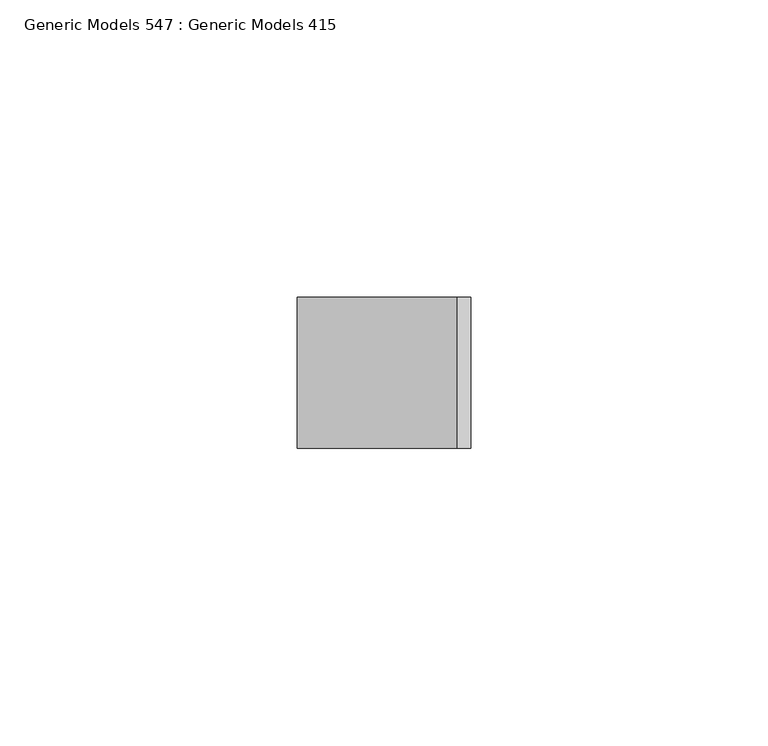
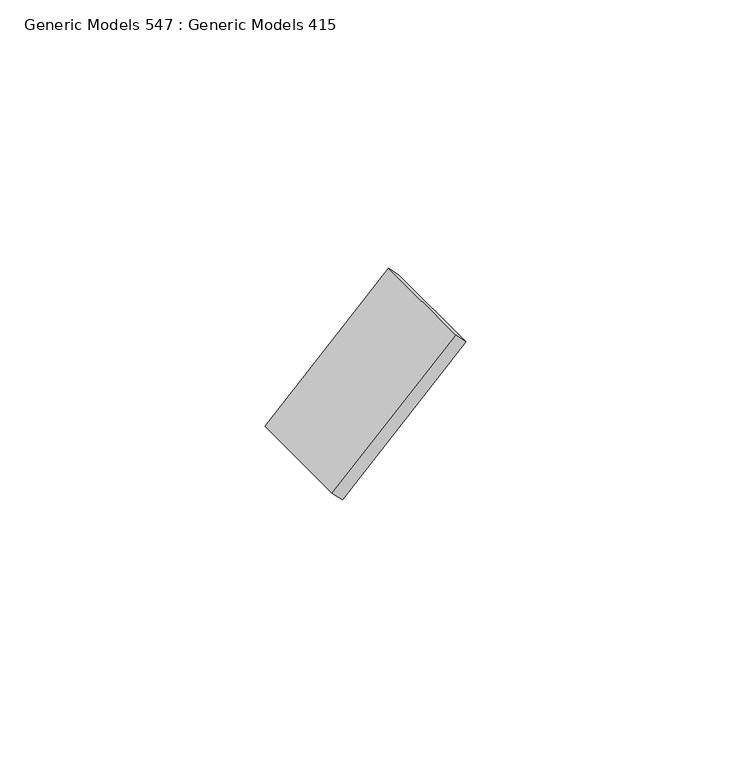
"""IFC4 building model written with IfcOpenShell, lengths in millimetres: proxy geometry, Generic Models 547 : Generic Models 415."""

from ifc_helpers import new_model, si_unit, frame, origin, place, context, project, spatial, polyline, outline, extrude, source, transform, mapped, element, save


def generic_models_547_generic_models_415_fd695bb7(model_context):
    return source(origin(), model_context, "Body", "SweptSolid", [
        extrude(outline(polyline([(0.0, -3.175), (0.0, 0.0), (25.4, 0.0), (25.4, -3.175), (0.0, -3.175)])), frame((7848.0411784, 4501.3863946, 124813.3849742), z_axis=(0.7071067811867181, 0.0, 0.707106781186377), x_axis=(0.0, -1.0, 0.0)), (0.0, 0.0, 1.0), 38.1),
    ])


if __name__ == "__main__":
    model = new_model("IFC4")
    model_context = context("Model", 3, world=origin())
    ifc_project = project(units=[si_unit("LENGTHUNIT", "METRE", prefix="MILLI")], contexts=[model_context])
    site = spatial("IfcSite", under=ifc_project)
    building = spatial("IfcBuilding", under=site)
    placement = place(None, origin())
    generic_models_547_generic_models_415_shape = generic_models_547_generic_models_415_fd695bb7(model_context)
    element("IfcBuildingElementProxy", 1, Name="Generic Models 547 : Generic Models 415", ObjectType="Generic Models 547 : Generic Models 415", at=placement, inside=building, context=model_context, shape_type="MappedRepresentation", body=[
        mapped(generic_models_547_generic_models_415_shape, transform((0.0, 0.0, 0.0), x_axis=(1.0, 0.0, 0.0), y_axis=(0.0, 1.0, 0.0), z_axis=(0.0, 0.0, 1.0))),
    ])
    save(model, "model.ifc")

# Revit data of these elements
# Element 1 (IfcBuildingElementProxy, "Generic Models 547 : Generic Models 415")
#   Materials on its faces: "_WELDED STEEL TABS FOR LOUVER ATTACHMENT"
# Materials
#   "_WELDED STEEL TABS FOR LOUVER ATTACHMENT": class "Metal", colour RGB 199 199 199, transparency 0, Description = "Structural steel 50ksi", Cost = 0
